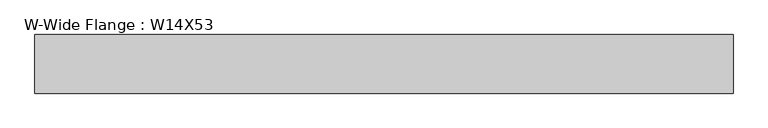
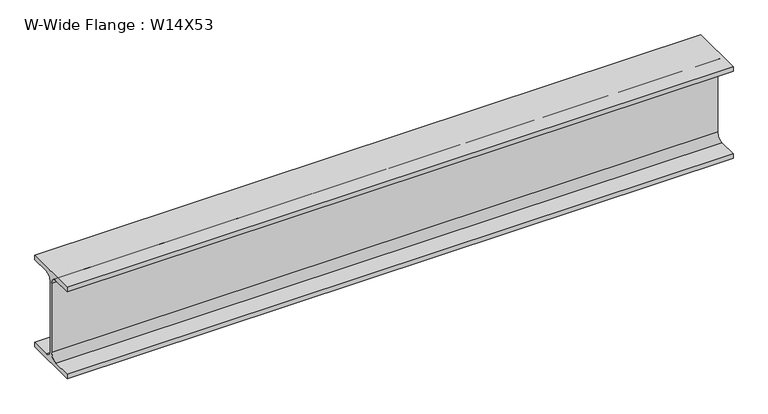
"""IFC4 building model written with IfcOpenShell, lengths in millimetres: beam geometry, W-Wide Flange : W14X53."""

import ifcopenshell
import ifcopenshell.guid

model = None  # the IFC model being written
_history = None  # IfcOwnerHistory: only IFC2X3 demands one
_inside = {}  # id of a spatial element -> (the spatial element, [elements in it])
_under = {}  # id of a project, library or spatial element -> (it, [spatial elements below it])
_declared = {}  # id of a project -> (the project, [libraries it declares])
_typed = {}  # id of a type object -> (the type object, [elements of that type])
_made_of = {}  # id of a material, layer set ... -> (it, [elements and type objects made of it])


def new_model(schema):
    """Start an empty IFC model of exactly this schema.

    Asked for "IFC4X3", IfcOpenShell would pick the latest addendum, in which some entities
    have other attributes; the version numbers below select the first issue.
    IFC2X3 requires an IfcOwnerHistory on every rooted entity: one is made here for all.
    """
    global model, _history
    if schema == "IFC4X3":
        model = ifcopenshell.file(schema_version=(4, 3, 0, 0))
    else:
        model = ifcopenshell.file(schema=schema)
    _inside.clear()
    _under.clear()
    _declared.clear()
    _typed.clear()
    _made_of.clear()
    _history = None
    if model.schema == "IFC2X3":
        org = make("IfcOrganization", Name="unknown")
        user = make(
            "IfcPersonAndOrganization",
            ThePerson=make("IfcPerson", FamilyName="unknown"),
            TheOrganization=org,
        )
        app = make(
            "IfcApplication",
            ApplicationDeveloper=org,
            Version="unknown",
            ApplicationFullName="unknown",
            ApplicationIdentifier="unknown",
        )
        _history = make(
            "IfcOwnerHistory",
            OwningUser=user,
            OwningApplication=app,
            ChangeAction="ADDED",
            CreationDate=0,
        )
    return model


def make(cls, **values):
    """One entity of the class cls with the attributes given. An attribute that is None is left unset."""
    return model.create_entity(
        cls, **{name: value for name, value in values.items() if value is not None}
    )


def rooted(cls, **values):
    """An entity with a GlobalId (a new one), such as an element, a storey or a relation."""
    return make(cls, GlobalId=ifcopenshell.guid.new(), OwnerHistory=_history, **values)


def si_unit(unit_type, name, prefix=None):
    """IfcSIUnit, for example si_unit("LENGTHUNIT", "METRE", prefix="MILLI")."""
    return make("IfcSIUnit", UnitType=unit_type, Prefix=prefix, Name=name)


def assignment(units):
    """IfcUnitAssignment: the units of a project."""
    return None if units is None else make("IfcUnitAssignment", Units=units)


def point(xyz):
    """IfcCartesianPoint."""
    return None if xyz is None else make("IfcCartesianPoint", Coordinates=xyz)


def direction(xyz):
    """IfcDirection."""
    return None if xyz is None else make("IfcDirection", DirectionRatios=xyz)


def frame(location, z_axis=None, x_axis=None):
    """IfcAxis2Placement3D, a coordinate frame: its origin and axes. An axis left out is left unset."""
    return make(
        "IfcAxis2Placement3D",
        Location=point(location),
        Axis=direction(z_axis),
        RefDirection=direction(x_axis),
    )


def frame_2d(location, x_axis=None):
    """IfcAxis2Placement2D, a coordinate frame in the plane: its origin and x axis."""
    return make(
        "IfcAxis2Placement2D", Location=point(location), RefDirection=direction(x_axis)
    )


def origin():
    """The frame at (0, 0, 0) with its axes left unset."""
    return frame((0.0, 0.0, 0.0))


def place(relative_to, where):
    """IfcLocalPlacement: puts the frame where relative to a parent placement (None: the world)."""
    return make(
        "IfcLocalPlacement", PlacementRelTo=relative_to, RelativePlacement=where
    )


def context(
    kind, dimensions, precision=None, world=None, true_north=None, identifier=None
):
    """IfcGeometricRepresentationContext, for example the 3D "Model" context."""
    return make(
        "IfcGeometricRepresentationContext",
        ContextIdentifier=identifier,
        ContextType=kind,
        CoordinateSpaceDimension=dimensions,
        Precision=precision,
        WorldCoordinateSystem=world,
        TrueNorth=true_north,
    )


def project(units=None, contexts=None):
    """IfcProject with its units and contexts."""
    return rooted(
        "IfcProject",
        Name="project",
        RepresentationContexts=contexts,
        UnitsInContext=assignment(units),
    )


def spatial(cls, under=None, at=None, **own):
    """A site, building, storey or space (cls), placed at a placement, below another one or the project."""
    s = rooted(cls, ObjectPlacement=at, **own)
    if under is not None:
        _under.setdefault(under.id(), (under, []))[1].append(s)
    return s


def polyline(points):
    """IfcPolyline through the points."""
    return make("IfcPolyline", Points=[point(p) for p in points])


def circle_curve(where, radius):
    """IfcCircle in the frame where."""
    return make("IfcCircle", Position=where, Radius=radius)


def trimmed(basis, trim1, trim2, sense, master):
    """IfcTrimmedCurve: the piece of a basis curve between two trims."""
    return make(
        "IfcTrimmedCurve",
        BasisCurve=basis,
        Trim1=trim1,
        Trim2=trim2,
        SenseAgreement=sense,
        MasterRepresentation=master,
    )


def segment(curve, same_sense, transition):
    """IfcCompositeCurveSegment."""
    return make(
        "IfcCompositeCurveSegment",
        Transition=transition,
        SameSense=same_sense,
        ParentCurve=curve,
    )


def composite_curve(segments, self_intersect=None):
    """IfcCompositeCurve: segments joined end to end."""
    return make("IfcCompositeCurve", Segments=segments, SelfIntersect=self_intersect)


def outline(outer, holes=None, kind="AREA"):
    """IfcArbitraryClosedProfileDef: a profile drawn as a closed curve; with holes, ...WithVoids."""
    if holes is None:
        return make("IfcArbitraryClosedProfileDef", ProfileType=kind, OuterCurve=outer)
    return make(
        "IfcArbitraryProfileDefWithVoids",
        ProfileType=kind,
        OuterCurve=outer,
        InnerCurves=holes,
    )


def extrude(swept, where, along, depth):
    """IfcExtrudedAreaSolid: the profile swept, set in the frame where, extruded along a direction by depth."""
    return make(
        "IfcExtrudedAreaSolid",
        SweptArea=swept,
        Position=where,
        ExtrudedDirection=direction(along),
        Depth=depth,
    )


def shape(context_of_items, identifier, shape_type, items):
    """IfcShapeRepresentation: the items that make up one representation, for example the "Body"."""
    return make(
        "IfcShapeRepresentation",
        ContextOfItems=context_of_items,
        RepresentationIdentifier=identifier,
        RepresentationType=shape_type,
        Items=items,
    )


def source(mapping_origin, context_of_items, identifier, shape_type, items):
    """IfcRepresentationMap: a shape defined once, which mapped items show again and again."""
    return make(
        "IfcRepresentationMap",
        MappingOrigin=mapping_origin,
        MappedRepresentation=shape(context_of_items, identifier, shape_type, items),
    )


def transform(
    local_origin,
    x_axis=None,
    y_axis=None,
    z_axis=None,
    scale=None,
    scale2=None,
    scale3=None,
    uniform=True,
):
    """IfcCartesianTransformationOperator3D, or its non-uniform kind. x_axis, y_axis, z_axis: its Axis1, 2, 3."""
    if uniform:
        return make(
            "IfcCartesianTransformationOperator3D",
            Axis1=direction(x_axis),
            Axis2=direction(y_axis),
            LocalOrigin=point(local_origin),
            Scale=scale,
            Axis3=direction(z_axis),
        )
    return make(
        "IfcCartesianTransformationOperator3DnonUniform",
        Axis1=direction(x_axis),
        Axis2=direction(y_axis),
        LocalOrigin=point(local_origin),
        Scale=scale,
        Axis3=direction(z_axis),
        Scale2=scale2,
        Scale3=scale3,
    )


def mapped(mapping_source, mapping_target):
    """IfcMappedItem: shows the shape of a source again, moved by a transform."""
    return make(
        "IfcMappedItem", MappingSource=mapping_source, MappingTarget=mapping_target
    )


def made_of(thing, what):
    """Note that an element or type object is made of a material, layer set ...; save() writes the relation."""
    if what is not None:
        _made_of.setdefault(what.id(), (what, []))[1].append(thing)
    return thing


def element(
    cls,
    number,
    at=None,
    inside=None,
    cuts=None,
    type_object=None,
    material=None,
    context=None,
    identifier="Body",
    shape_type=None,
    held_by="IfcProductDefinitionShape",
    body=None,
    shapes=None,
    **own,
):
    """One element of the class cls, such as IfcWall. Its Tag is "e" and its number.

    at: its placement. inside: the storey or other place that contains it. cuts: it is an
    opening in that element (IfcRelVoidsElement). A single representation is given by context,
    identifier, shape_type and body (its items); several are given by shapes. held_by: the class
    of the entity that holds the representations. save() writes the other relations.
    """
    e = rooted(cls, Tag="e%d" % number, ObjectPlacement=at, **own)
    if body is not None:
        shapes = [shape(context, identifier, shape_type, body)]
    if shapes is not None:
        e.Representation = make(held_by, Representations=shapes)
    if inside is not None:
        _inside.setdefault(inside.id(), (inside, []))[1].append(e)
    if cuts is not None:
        rooted(
            "IfcRelVoidsElement", RelatingBuildingElement=cuts, RelatedOpeningElement=e
        )
    if type_object is not None:
        _typed.setdefault(type_object.id(), (type_object, []))[1].append(e)
    return made_of(e, material)


def aggregate(whole, parts):
    """IfcRelAggregates: a whole, such as a stair, and the parts it consists of."""
    return rooted("IfcRelAggregates", RelatingObject=whole, RelatedObjects=parts)


def save(model, path):
    """Write the relations noted so far, then the file.

    IfcRelAggregates (storeys below a building ...), IfcRelContainedInSpatialStructure (elements
    in a storey), IfcRelDefinesByType, IfcRelAssociatesMaterial and IfcRelDeclares: one each for
    every whole, place, type object, material and project.
    """
    for whole, parts in _under.values():
        aggregate(whole, parts)
    for where, things in _inside.values():
        rooted(
            "IfcRelContainedInSpatialStructure",
            RelatedElements=things,
            RelatingStructure=where,
        )
    for kind, things in _typed.values():
        rooted("IfcRelDefinesByType", RelatedObjects=things, RelatingType=kind)
    for what, things in _made_of.values():
        rooted("IfcRelAssociatesMaterial", RelatedObjects=things, RelatingMaterial=what)
    for by, libraries in _declared.values():
        rooted("IfcRelDeclares", RelatingContext=by, RelatedDefinitions=libraries)
    model.write(path)


def w_wide_flange_w14x53_735d448f(model_context):
    return source(origin(), model_context, "Body", "SweptSolid", [
        extrude(outline(composite_curve([segment(polyline([(102.3441406, -160.0398438), (102.3441406, -176.8078125), (-102.3441406, -176.8078125), (-102.3441406, -160.0398438), (-30.8074219, -160.0398438)]), True, "CONTINUOUS"), segment(trimmed(circle_curve(frame_2d((-30.8074219, -133.9453125)), 26.0945313), [point((-30.8074219, -160.0398438))], [point((-4.7128906, -133.9453125))], True, "CARTESIAN"), True, "CONTINUOUS"), segment(polyline([(-4.7128906, -133.9453125), (-4.7128906, 133.9453125)]), True, "CONTINUOUS"), segment(trimmed(circle_curve(frame_2d((-30.8074219, 133.9453125)), 26.0945313), [point((-4.7128906, 133.9453125))], [point((-30.8074219, 160.0398437))], True, "CARTESIAN"), True, "CONTINUOUS"), segment(polyline([(-30.8074219, 160.0398437), (-102.3441406, 160.0398437), (-102.3441406, 176.8078125), (102.3441406, 176.8078125), (102.3441406, 160.0398437), (30.8074219, 160.0398437)]), True, "CONTINUOUS"), segment(trimmed(circle_curve(frame_2d((30.8074219, 133.9453125)), 26.0945312), [point((30.8074219, 160.0398437))], [point((4.7128906, 133.9453125))], True, "CARTESIAN"), True, "CONTINUOUS"), segment(polyline([(4.7128906, 133.9453125), (4.7128906, -133.9453125)]), True, "CONTINUOUS"), segment(trimmed(circle_curve(frame_2d((30.8074219, -133.9453125)), 26.0945313), [point((4.7128906, -133.9453125))], [point((30.8074219, -160.0398438))], True, "CARTESIAN"), True, "CONTINUOUS"), segment(polyline([(30.8074219, -160.0398438), (102.3441406, -160.0398438)]), True, "CONTINUOUS")], self_intersect=False)), frame((-1219.327, 0.0, 0.0), z_axis=(1.0, 0.0, 0.0), x_axis=(0.0, 1.0, 0.0)), (0.0, 0.0, 1.0), 2438.654),
    ])


if __name__ == "__main__":
    model = new_model("IFC4")
    model_context = context("Model", 3, world=origin())
    ifc_project = project(units=[si_unit("LENGTHUNIT", "METRE", prefix="MILLI")], contexts=[model_context])
    site = spatial("IfcSite", under=ifc_project)
    building = spatial("IfcBuilding", under=site)
    placement = place(None, origin())
    w_wide_flange_w14x53_shape = w_wide_flange_w14x53_735d448f(model_context)
    element("IfcBeam", 1, ObjectType="W-Wide Flange : W14X53", at=placement, inside=building, context=model_context, shape_type="MappedRepresentation", body=[
        mapped(w_wide_flange_w14x53_shape, transform((0.0, 0.0, 0.0), x_axis=(1.0, 0.0, 0.0), y_axis=(0.0, 1.0, 0.0), z_axis=(0.0, 0.0, 1.0))),
    ])
    save(model, "model.ifc")

# Revit data of these elements
# Type "W-Wide Flange : W14X53"
#   Assembly Code = "B10"
#   W = 52
#   Length [instance default] = 5' - 0"
#   bf = 0' - 8 15/256"
#   d = 1' - 1 59/64"
#   k = 0' - 1 11/16"
#   k2 = 0' - 1 7/256"
#   tf = 0' - 0 169/256"
#   tw = 0' - 0 95/256"
#   A = 0.166667 SF
#   Structural Material [instance default] = _STRUCTURAL STEEL (SEE STRUCT. DWGS)
# Element 1 (IfcBeam, "W-Wide Flange : W14X53")
#   Materials on its faces: "_STRUCTURAL STEEL (SEE STRUCT. DWGS)"
# Materials
#   "_STRUCTURAL STEEL (SEE STRUCT. DWGS)": class "Metal", colour RGB 199 199 199, transparency 0, Description = "Structural steel 50ksi", Cost = 0
